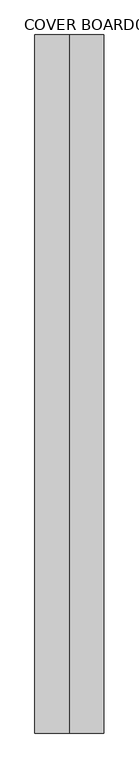
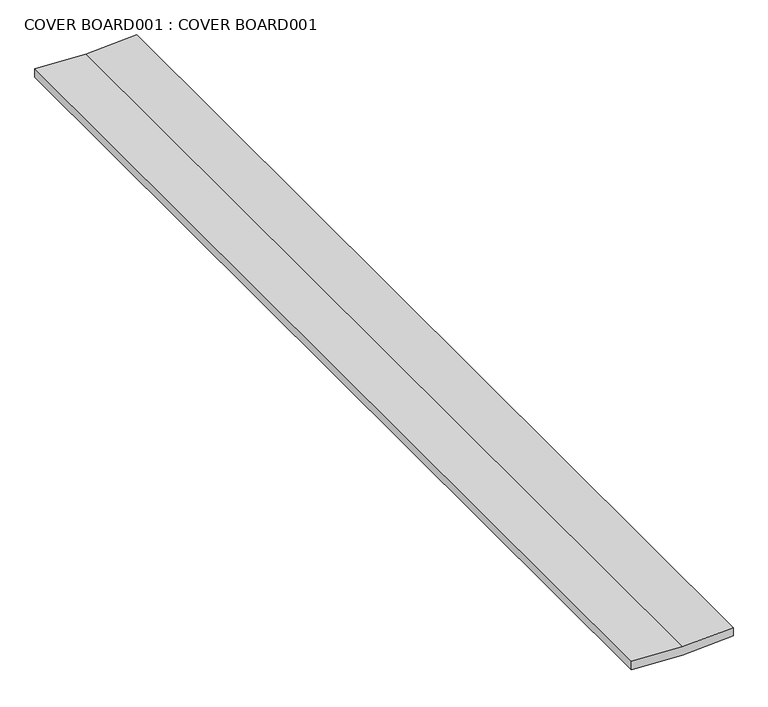
"""IFC4 building model written with IfcOpenShell, lengths in millimetres: proxy geometry, COVER BOARD001 : COVER BOARD001."""

from ifc_helpers import new_model, si_unit, frame, origin, place, context, project, spatial, polyline, outline, extrude, source, transform, mapped, element, save


def cover_board001_cover_board001_2390c736(model_context):
    return source(origin(), model_context, "Body", "SweptSolid", [
        extrude(outline(polyline([(40228.3444286, -4699.8063764), (40233.346, -4797.9038825), (40216.0142809, -4797.9038825), (40211.0127094, -4699.8063764), (40216.0142809, -4601.0538825), (40233.346, -4601.0538825), (40228.3444286, -4699.8063764)])), frame((0.0, -1052.6406573, 0.0), z_axis=(0.0, 1.0, 0.0), x_axis=(0.0, 0.0, 1.0)), (0.0, 0.0, 1.0), 2000.0),
    ])


if __name__ == "__main__":
    model = new_model("IFC4")
    model_context = context("Model", 3, world=origin())
    ifc_project = project(units=[si_unit("LENGTHUNIT", "METRE", prefix="MILLI")], contexts=[model_context])
    site = spatial("IfcSite", under=ifc_project)
    building = spatial("IfcBuilding", under=site)
    placement = place(None, origin())
    cover_board001_cover_board001_shape = cover_board001_cover_board001_2390c736(model_context)
    element("IfcBuildingElementProxy", 1, Name="COVER BOARD001 : COVER BOARD001", ObjectType="COVER BOARD001 : COVER BOARD001", at=placement, inside=building, context=model_context, shape_type="MappedRepresentation", body=[
        mapped(cover_board001_cover_board001_shape, transform((0.0, 0.0, 0.0), x_axis=(1.0, 0.0, 0.0), y_axis=(0.0, 1.0, 0.0), z_axis=(0.0, 0.0, 1.0))),
    ])
    save(model, "model.ifc")

# Revit data of these elements
# Type "COVER BOARD001 : COVER BOARD001"
#   NameOverride = "COVER BOARD001"
# Element 1 (IfcBuildingElementProxy, "COVER BOARD001 : COVER BOARD001")
#   Materials on its faces: "CDX PLYWOOD - SEE STRUCTURAL DWGS"
# Materials
#   "CDX PLYWOOD - SEE STRUCTURAL DWGS": class "Unassigned", colour RGB 202 163 108, transparency 0, Cost = 0
